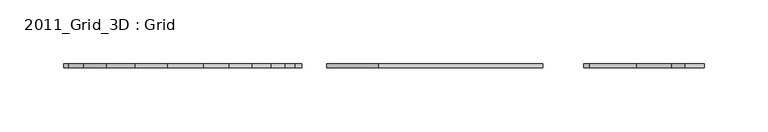
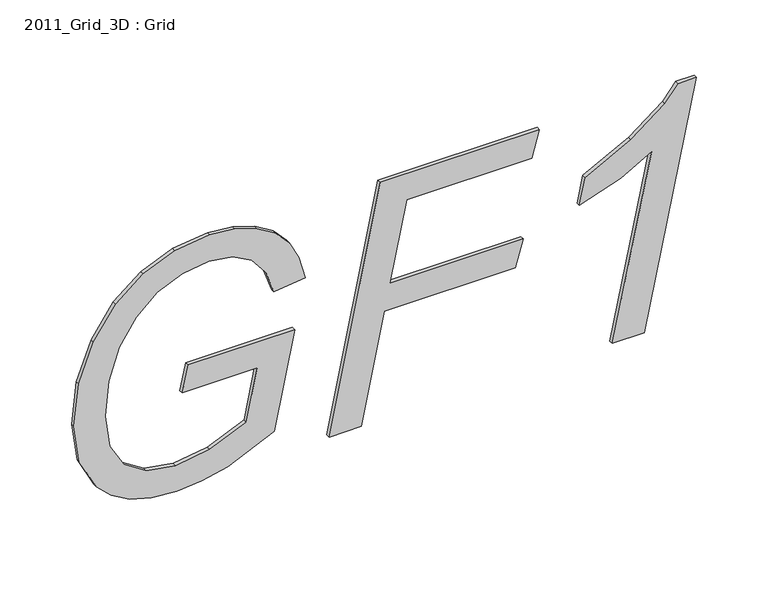
"""IFC4 building model written with IfcOpenShell, lengths in millimetres: proxy geometry, 2011_Grid_3D : Grid."""

import ifcopenshell
import ifcopenshell.guid

model = None  # the IFC model being written
_history = None  # IfcOwnerHistory: only IFC2X3 demands one
_inside = {}  # id of a spatial element -> (the spatial element, [elements in it])
_under = {}  # id of a project, library or spatial element -> (it, [spatial elements below it])
_declared = {}  # id of a project -> (the project, [libraries it declares])
_typed = {}  # id of a type object -> (the type object, [elements of that type])
_made_of = {}  # id of a material, layer set ... -> (it, [elements and type objects made of it])


def new_model(schema):
    """Start an empty IFC model of exactly this schema.

    Asked for "IFC4X3", IfcOpenShell would pick the latest addendum, in which some entities
    have other attributes; the version numbers below select the first issue.
    IFC2X3 requires an IfcOwnerHistory on every rooted entity: one is made here for all.
    """
    global model, _history
    if schema == "IFC4X3":
        model = ifcopenshell.file(schema_version=(4, 3, 0, 0))
    else:
        model = ifcopenshell.file(schema=schema)
    _inside.clear()
    _under.clear()
    _declared.clear()
    _typed.clear()
    _made_of.clear()
    _history = None
    if model.schema == "IFC2X3":
        org = make("IfcOrganization", Name="unknown")
        user = make(
            "IfcPersonAndOrganization",
            ThePerson=make("IfcPerson", FamilyName="unknown"),
            TheOrganization=org,
        )
        app = make(
            "IfcApplication",
            ApplicationDeveloper=org,
            Version="unknown",
            ApplicationFullName="unknown",
            ApplicationIdentifier="unknown",
        )
        _history = make(
            "IfcOwnerHistory",
            OwningUser=user,
            OwningApplication=app,
            ChangeAction="ADDED",
            CreationDate=0,
        )
    return model


def make(cls, **values):
    """One entity of the class cls with the attributes given. An attribute that is None is left unset."""
    return model.create_entity(
        cls, **{name: value for name, value in values.items() if value is not None}
    )


def rooted(cls, **values):
    """An entity with a GlobalId (a new one), such as an element, a storey or a relation."""
    return make(cls, GlobalId=ifcopenshell.guid.new(), OwnerHistory=_history, **values)


def si_unit(unit_type, name, prefix=None):
    """IfcSIUnit, for example si_unit("LENGTHUNIT", "METRE", prefix="MILLI")."""
    return make("IfcSIUnit", UnitType=unit_type, Prefix=prefix, Name=name)


def assignment(units):
    """IfcUnitAssignment: the units of a project."""
    return None if units is None else make("IfcUnitAssignment", Units=units)


def point(xyz):
    """IfcCartesianPoint."""
    return None if xyz is None else make("IfcCartesianPoint", Coordinates=xyz)


def direction(xyz):
    """IfcDirection."""
    return None if xyz is None else make("IfcDirection", DirectionRatios=xyz)


def frame(location, z_axis=None, x_axis=None):
    """IfcAxis2Placement3D, a coordinate frame: its origin and axes. An axis left out is left unset."""
    return make(
        "IfcAxis2Placement3D",
        Location=point(location),
        Axis=direction(z_axis),
        RefDirection=direction(x_axis),
    )


def origin():
    """The frame at (0, 0, 0) with its axes left unset."""
    return frame((0.0, 0.0, 0.0))


def place(relative_to, where):
    """IfcLocalPlacement: puts the frame where relative to a parent placement (None: the world)."""
    return make(
        "IfcLocalPlacement", PlacementRelTo=relative_to, RelativePlacement=where
    )


def context(
    kind, dimensions, precision=None, world=None, true_north=None, identifier=None
):
    """IfcGeometricRepresentationContext, for example the 3D "Model" context."""
    return make(
        "IfcGeometricRepresentationContext",
        ContextIdentifier=identifier,
        ContextType=kind,
        CoordinateSpaceDimension=dimensions,
        Precision=precision,
        WorldCoordinateSystem=world,
        TrueNorth=true_north,
    )


def project(units=None, contexts=None):
    """IfcProject with its units and contexts."""
    return rooted(
        "IfcProject",
        Name="project",
        RepresentationContexts=contexts,
        UnitsInContext=assignment(units),
    )


def spatial(cls, under=None, at=None, **own):
    """A site, building, storey or space (cls), placed at a placement, below another one or the project."""
    s = rooted(cls, ObjectPlacement=at, **own)
    if under is not None:
        _under.setdefault(under.id(), (under, []))[1].append(s)
    return s


def polyline(points):
    """IfcPolyline through the points."""
    return make("IfcPolyline", Points=[point(p) for p in points])


def outline(outer, holes=None, kind="AREA"):
    """IfcArbitraryClosedProfileDef: a profile drawn as a closed curve; with holes, ...WithVoids."""
    if holes is None:
        return make("IfcArbitraryClosedProfileDef", ProfileType=kind, OuterCurve=outer)
    return make(
        "IfcArbitraryProfileDefWithVoids",
        ProfileType=kind,
        OuterCurve=outer,
        InnerCurves=holes,
    )


def extrude(swept, where, along, depth):
    """IfcExtrudedAreaSolid: the profile swept, set in the frame where, extruded along a direction by depth."""
    return make(
        "IfcExtrudedAreaSolid",
        SweptArea=swept,
        Position=where,
        ExtrudedDirection=direction(along),
        Depth=depth,
    )


def shape(context_of_items, identifier, shape_type, items):
    """IfcShapeRepresentation: the items that make up one representation, for example the "Body"."""
    return make(
        "IfcShapeRepresentation",
        ContextOfItems=context_of_items,
        RepresentationIdentifier=identifier,
        RepresentationType=shape_type,
        Items=items,
    )


def source(mapping_origin, context_of_items, identifier, shape_type, items):
    """IfcRepresentationMap: a shape defined once, which mapped items show again and again."""
    return make(
        "IfcRepresentationMap",
        MappingOrigin=mapping_origin,
        MappedRepresentation=shape(context_of_items, identifier, shape_type, items),
    )


def transform(
    local_origin,
    x_axis=None,
    y_axis=None,
    z_axis=None,
    scale=None,
    scale2=None,
    scale3=None,
    uniform=True,
):
    """IfcCartesianTransformationOperator3D, or its non-uniform kind. x_axis, y_axis, z_axis: its Axis1, 2, 3."""
    if uniform:
        return make(
            "IfcCartesianTransformationOperator3D",
            Axis1=direction(x_axis),
            Axis2=direction(y_axis),
            LocalOrigin=point(local_origin),
            Scale=scale,
            Axis3=direction(z_axis),
        )
    return make(
        "IfcCartesianTransformationOperator3DnonUniform",
        Axis1=direction(x_axis),
        Axis2=direction(y_axis),
        LocalOrigin=point(local_origin),
        Scale=scale,
        Axis3=direction(z_axis),
        Scale2=scale2,
        Scale3=scale3,
    )


def mapped(mapping_source, mapping_target):
    """IfcMappedItem: shows the shape of a source again, moved by a transform."""
    return make(
        "IfcMappedItem", MappingSource=mapping_source, MappingTarget=mapping_target
    )


def made_of(thing, what):
    """Note that an element or type object is made of a material, layer set ...; save() writes the relation."""
    if what is not None:
        _made_of.setdefault(what.id(), (what, []))[1].append(thing)
    return thing


def element(
    cls,
    number,
    at=None,
    inside=None,
    cuts=None,
    type_object=None,
    material=None,
    context=None,
    identifier="Body",
    shape_type=None,
    held_by="IfcProductDefinitionShape",
    body=None,
    shapes=None,
    **own,
):
    """One element of the class cls, such as IfcWall. Its Tag is "e" and its number.

    at: its placement. inside: the storey or other place that contains it. cuts: it is an
    opening in that element (IfcRelVoidsElement). A single representation is given by context,
    identifier, shape_type and body (its items); several are given by shapes. held_by: the class
    of the entity that holds the representations. save() writes the other relations.
    """
    e = rooted(cls, Tag="e%d" % number, ObjectPlacement=at, **own)
    if body is not None:
        shapes = [shape(context, identifier, shape_type, body)]
    if shapes is not None:
        e.Representation = make(held_by, Representations=shapes)
    if inside is not None:
        _inside.setdefault(inside.id(), (inside, []))[1].append(e)
    if cuts is not None:
        rooted(
            "IfcRelVoidsElement", RelatingBuildingElement=cuts, RelatedOpeningElement=e
        )
    if type_object is not None:
        _typed.setdefault(type_object.id(), (type_object, []))[1].append(e)
    return made_of(e, material)


def aggregate(whole, parts):
    """IfcRelAggregates: a whole, such as a stair, and the parts it consists of."""
    return rooted("IfcRelAggregates", RelatingObject=whole, RelatedObjects=parts)


def save(model, path):
    """Write the relations noted so far, then the file.

    IfcRelAggregates (storeys below a building ...), IfcRelContainedInSpatialStructure (elements
    in a storey), IfcRelDefinesByType, IfcRelAssociatesMaterial and IfcRelDeclares: one each for
    every whole, place, type object, material and project.
    """
    for whole, parts in _under.values():
        aggregate(whole, parts)
    for where, things in _inside.values():
        rooted(
            "IfcRelContainedInSpatialStructure",
            RelatedElements=things,
            RelatingStructure=where,
        )
    for kind, things in _typed.values():
        rooted("IfcRelDefinesByType", RelatedObjects=things, RelatingType=kind)
    for what, things in _made_of.values():
        rooted("IfcRelAssociatesMaterial", RelatedObjects=things, RelatingMaterial=what)
    for by, libraries in _declared.values():
        rooted("IfcRelDeclares", RelatingContext=by, RelatedDefinitions=libraries)
    model.write(path)


def proxy_2011_grid_3d_grid_895aad00(model_context):
    return source(origin(), model_context, "Body", "SweptSolid", [
        extrude(outline(polyline([(-22.2856526, 47336.5225939), (-22.2856526, 47396.9997838), (-65.3632575, 47388.324777), (-78.2642318, 47358.8049683), (-82.5645566, 47331.3175898), (-78.6484107, 47307.5728571), (-66.899973, 47289.5784145), (-47.5051365, 47278.2389414), (-20.6497942, 47274.459117), (8.448657, 47277.3280657), (34.2753914, 47285.9349117), (55.4114257, 47299.3377971), (70.4377767, 47316.5948641), (79.4164087, 47336.510201), (82.409286, 47357.8878962), (79.5465338, 47377.2269648), (70.9582771, 47392.7118519), (56.9915162, 47403.9583785), (37.9932514, 47410.5823658), (41.1658253, 47435.9629569), (60.4119475, 47430.7393636), (75.617995, 47423.0000183), (87.4841649, 47412.0261347), (96.7106543, 47397.0989267), (102.640641, 47379.0920913), (104.6173033, 47358.8793255), (101.0419612, 47330.6297857), (90.315935, 47305.069498), (72.1170101, 47282.9358379), (46.1229721, 47264.9661811), (14.5831261, 47253.0504396), (-20.2532224, 47249.0785258), (-52.387926, 47253.5895294), (-78.1031246, 47267.1225399), (-89.7710087, 47279.2303707), (-98.1052116, 47294.089418), (-103.1057333, 47311.6996817), (-104.7725739, 47332.0611618), (-103.1243226, 47352.5713564), (-98.1795688, 47373.4533369), (-81.1765555, 47410.929366), (-0.0776353, 47427.3375217), (-0.0776353, 47341.4301691), (-22.2856526, 47336.5225939)])), frame((0.0, -3.175, 0.0), z_axis=(0.0, 1.0, 0.0), x_axis=(0.0, 0.0, 1.0)), (0.0, 0.0, 1.0), 3.175),
        extrude(outline(polyline([(-101.6, 47455.2958291), (-101.6, 47481.072992), (-9.595357, 47499.6622922), (-9.595357, 47605.4973745), (12.6126603, 47611.8425223), (12.6126603, 47504.1732957), (79.2367121, 47517.6567348), (79.2367121, 47618.5842419), (101.4447294, 47624.9293897), (101.4447294, 47496.3410039), (-101.6, 47455.2958291)])), frame((0.0, -3.175, 0.0), z_axis=(0.0, 1.0, 0.0), x_axis=(0.0, 0.0, 1.0)), (0.0, 0.0, 1.0), 3.175),
        extrude(outline(polyline([(-101.6, 47683.7211497), (-101.6, 47709.547884), (101.4447294, 47751.7332026), (101.4447294, 47736.9113339), (88.0108618, 47726.1543255), (67.0173455, 47698.7165185), (47.5109731, 47661.9592756), (25.3029559, 47657.2995577), (36.729179, 47690.574405), (51.3775476, 47715.4468886), (-101.6, 47683.7211497)])), frame((0.0, -3.175, 0.0), z_axis=(0.0, 1.0, 0.0), x_axis=(0.0, 0.0, 1.0)), (0.0, 0.0, 1.0), 3.175),
    ])


if __name__ == "__main__":
    model = new_model("IFC4")
    model_context = context("Model", 3, world=origin())
    ifc_project = project(units=[si_unit("LENGTHUNIT", "METRE", prefix="MILLI")], contexts=[model_context])
    site = spatial("IfcSite", under=ifc_project)
    building = spatial("IfcBuilding", under=site)
    placement = place(None, origin())
    proxy_2011_grid_3d_grid_shape = proxy_2011_grid_3d_grid_895aad00(model_context)
    element("IfcBuildingElementProxy", 1, Name="2011_Grid_3D : Grid", ObjectType="2011_Grid_3D : Grid", at=placement, inside=building, context=model_context, shape_type="MappedRepresentation", body=[
        mapped(proxy_2011_grid_3d_grid_shape, transform((0.0, 0.0, 0.0), x_axis=(1.0, 0.0, 0.0), y_axis=(0.0, 1.0, 0.0), z_axis=(0.0, 0.0, 1.0))),
    ])
    save(model, "model.ifc")

# Revit data of these elements
# Type "2011_Grid_3D : Grid"
#   Workplane [instance default] = "LEVEL"
#   Grid [instance default] = "S"
#   t [instance default] = 12' - 6"
#   built-in parameter 1001306 [instance default] = 50 (stored number, unit not read)
#   d [instance default] = 2
#   Symbol At End 2 [instance default] = yes
#   Symbol At End 1 [instance default] = yes
#   Robust [instance default] = yes
#   No of grid markers [instance default] = 3
#   Grid Height Visible = yes
#   Height = 0
#   Assembly Code = ""
# Element 1 (IfcBuildingElementProxy, "2011_Grid_3D : Grid")
#   Workplane = "GF1"
#   Grid = "A"
#   t = 11' - 0.37148"
#   built-in parameter 1001306 = 154.433 (stored number, unit not read)
#   d = 7
#   Robust = no
#   No of grid markers = 8
#   Materials on its faces: "Letter"
# Materials
#   "Letter": class "Unassigned", colour RGB 178 187 30, transparency 0, Comments = "Rendering appearance not upgraded "
